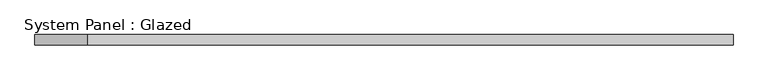
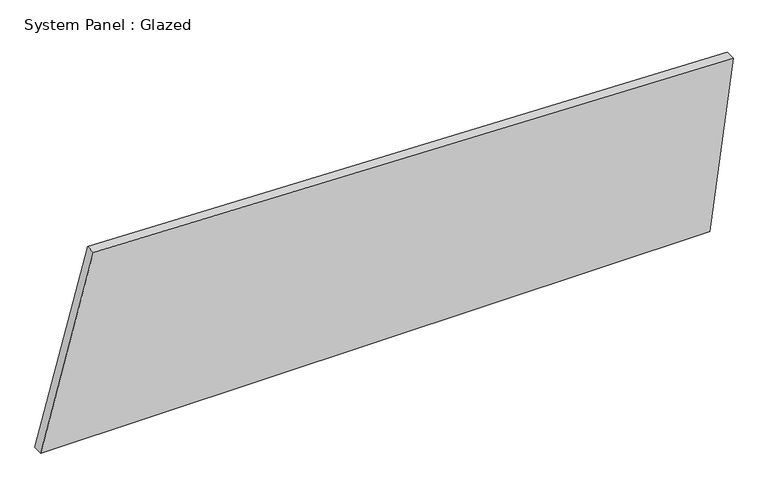
"""IFC4 building model written with IfcOpenShell, lengths in millimetres: plate geometry, System Panel : Glazed."""

from ifc_helpers import new_model, si_unit, frame, origin, place, context, project, spatial, polyline, outline, extrude, source, transform, mapped, element, save


def system_panel_glazed_24496e0b(model_context):
    return source(origin(), model_context, "Body", "SweptSolid", [
        extrude(outline(polyline([(0.0, -854.9177618), (0.0, 797.528072), (433.8154664, 854.9177618), (479.1651161, -724.9014664), (0.0, -854.9177618)])), frame((0.0, -49.5, 0.0), z_axis=(0.0, 1.0, 0.0), x_axis=(0.0, 0.0, 1.0)), (0.0, 0.0, 1.0), 25.0),
    ])


if __name__ == "__main__":
    model = new_model("IFC4")
    model_context = context("Model", 3, world=origin())
    ifc_project = project(units=[si_unit("LENGTHUNIT", "METRE", prefix="MILLI")], contexts=[model_context])
    site = spatial("IfcSite", under=ifc_project)
    building = spatial("IfcBuilding", under=site)
    placement = place(None, origin())
    system_panel_glazed_shape = system_panel_glazed_24496e0b(model_context)
    element("IfcPlate", 1, ObjectType="System Panel : Glazed", at=placement, inside=building, context=model_context, shape_type="MappedRepresentation", body=[
        mapped(system_panel_glazed_shape, transform((0.0, 0.0, 0.0), x_axis=(1.0, 0.0, 0.0), y_axis=(0.0, 1.0, 0.0), z_axis=(0.0, 0.0, 1.0))),
    ])
    save(model, "model.ifc")

# Revit data of these elements
# Element 1 (IfcPlate, "System Panel : Glazed")
#   Materials on its faces: "Glass, Clear Glazing"
# Materials
#   "Glass, Clear Glazing": class "Glass", colour RGB 247 249 248, transparency 0.85, Description = "Clear glazing", Cost = 0
